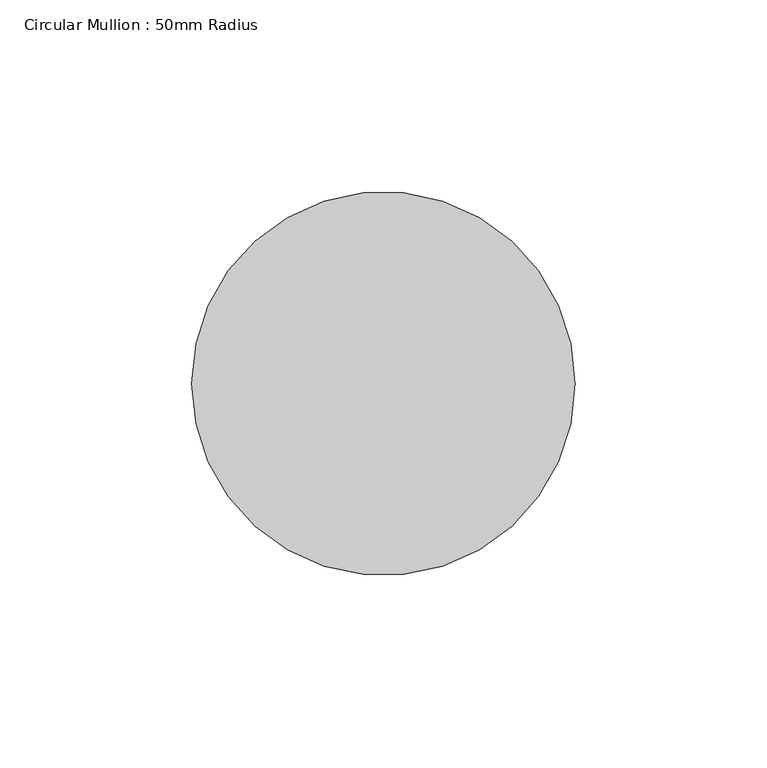
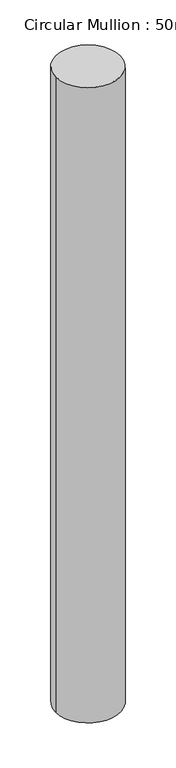
"""IFC4 building model written with IfcOpenShell, lengths in millimetres: member geometry, Circular Mullion : 50mm Radius."""

from ifc_helpers import new_model, si_unit, point, frame, origin, origin_2d, place, context, project, spatial, circle_curve, trimmed, segment, composite_curve, outline, extrude, source, transform, mapped, element, save


def circular_mullion_50mm_radius_c4641b67(model_context):
    return source(origin(), model_context, "Body", "SweptSolid", [
        extrude(outline(composite_curve([segment(trimmed(circle_curve(origin_2d(), 50.0), [point((50.0, 0.0))], [point((-50.0, 0.0))], False, "CARTESIAN"), True, "CONTINUOUS"), segment(trimmed(circle_curve(origin_2d(), 50.0), [point((-50.0, 0.0))], [point((50.0, 0.0))], False, "CARTESIAN"), True, "CONTINUOUS")], self_intersect=False)), frame((0.0, 0.0, -1043.6380657), z_axis=(0.0, 0.0, 1.0), x_axis=(1.0, 0.0, 0.0)), (0.0, 0.0, 1.0), 1043.6380657),
    ])


if __name__ == "__main__":
    model = new_model("IFC4")
    model_context = context("Model", 3, world=origin())
    ifc_project = project(units=[si_unit("LENGTHUNIT", "METRE", prefix="MILLI")], contexts=[model_context])
    site = spatial("IfcSite", under=ifc_project)
    building = spatial("IfcBuilding", under=site)
    placement = place(None, origin())
    circular_mullion_50mm_radius_shape = circular_mullion_50mm_radius_c4641b67(model_context)
    element("IfcMember", 1, ObjectType="Circular Mullion : 50mm Radius", at=placement, inside=building, context=model_context, shape_type="MappedRepresentation", body=[
        mapped(circular_mullion_50mm_radius_shape, transform((0.0, 0.0, 0.0), x_axis=(1.0, 0.0, 0.0), y_axis=(0.0, 1.0, 0.0), z_axis=(0.0, 0.0, 1.0))),
    ])
    save(model, "model.ifc")

# Revit data of these elements
# Type "Circular Mullion : 50mm Radius"
#   built-in parameter 1007350 = 0.164042 (stored number, unit not read)
# Element 1 (IfcMember, "Circular Mullion : 50mm Radius")
#   Materials on its faces: "Aluminium"
# Materials
#   "Aluminium": class "Metal", colour RGB 247 247 247, transparency 0, Description = "Aluminium 6061", Cost = 0
